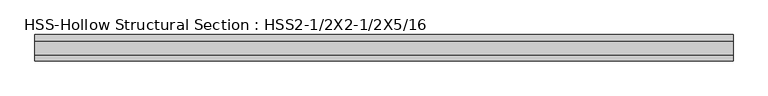
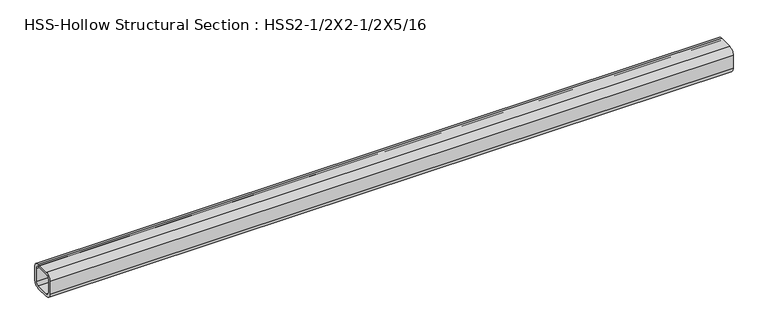
"""IFC4 building model written with IfcOpenShell, lengths in millimetres: beam geometry, HSS-Hollow Structural Section : HSS2-1/2X2-1/2X5/16."""

import ifcopenshell
import ifcopenshell.guid

model = None  # the IFC model being written
_history = None  # IfcOwnerHistory: only IFC2X3 demands one
_inside = {}  # id of a spatial element -> (the spatial element, [elements in it])
_under = {}  # id of a project, library or spatial element -> (it, [spatial elements below it])
_declared = {}  # id of a project -> (the project, [libraries it declares])
_typed = {}  # id of a type object -> (the type object, [elements of that type])
_made_of = {}  # id of a material, layer set ... -> (it, [elements and type objects made of it])


def new_model(schema):
    """Start an empty IFC model of exactly this schema.

    Asked for "IFC4X3", IfcOpenShell would pick the latest addendum, in which some entities
    have other attributes; the version numbers below select the first issue.
    IFC2X3 requires an IfcOwnerHistory on every rooted entity: one is made here for all.
    """
    global model, _history
    if schema == "IFC4X3":
        model = ifcopenshell.file(schema_version=(4, 3, 0, 0))
    else:
        model = ifcopenshell.file(schema=schema)
    _inside.clear()
    _under.clear()
    _declared.clear()
    _typed.clear()
    _made_of.clear()
    _history = None
    if model.schema == "IFC2X3":
        org = make("IfcOrganization", Name="unknown")
        user = make(
            "IfcPersonAndOrganization",
            ThePerson=make("IfcPerson", FamilyName="unknown"),
            TheOrganization=org,
        )
        app = make(
            "IfcApplication",
            ApplicationDeveloper=org,
            Version="unknown",
            ApplicationFullName="unknown",
            ApplicationIdentifier="unknown",
        )
        _history = make(
            "IfcOwnerHistory",
            OwningUser=user,
            OwningApplication=app,
            ChangeAction="ADDED",
            CreationDate=0,
        )
    return model


def make(cls, **values):
    """One entity of the class cls with the attributes given. An attribute that is None is left unset."""
    return model.create_entity(
        cls, **{name: value for name, value in values.items() if value is not None}
    )


def rooted(cls, **values):
    """An entity with a GlobalId (a new one), such as an element, a storey or a relation."""
    return make(cls, GlobalId=ifcopenshell.guid.new(), OwnerHistory=_history, **values)


def si_unit(unit_type, name, prefix=None):
    """IfcSIUnit, for example si_unit("LENGTHUNIT", "METRE", prefix="MILLI")."""
    return make("IfcSIUnit", UnitType=unit_type, Prefix=prefix, Name=name)


def assignment(units):
    """IfcUnitAssignment: the units of a project."""
    return None if units is None else make("IfcUnitAssignment", Units=units)


def point(xyz):
    """IfcCartesianPoint."""
    return None if xyz is None else make("IfcCartesianPoint", Coordinates=xyz)


def direction(xyz):
    """IfcDirection."""
    return None if xyz is None else make("IfcDirection", DirectionRatios=xyz)


def frame(location, z_axis=None, x_axis=None):
    """IfcAxis2Placement3D, a coordinate frame: its origin and axes. An axis left out is left unset."""
    return make(
        "IfcAxis2Placement3D",
        Location=point(location),
        Axis=direction(z_axis),
        RefDirection=direction(x_axis),
    )


def frame_2d(location, x_axis=None):
    """IfcAxis2Placement2D, a coordinate frame in the plane: its origin and x axis."""
    return make(
        "IfcAxis2Placement2D", Location=point(location), RefDirection=direction(x_axis)
    )


def origin():
    """The frame at (0, 0, 0) with its axes left unset."""
    return frame((0.0, 0.0, 0.0))


def place(relative_to, where):
    """IfcLocalPlacement: puts the frame where relative to a parent placement (None: the world)."""
    return make(
        "IfcLocalPlacement", PlacementRelTo=relative_to, RelativePlacement=where
    )


def context(
    kind, dimensions, precision=None, world=None, true_north=None, identifier=None
):
    """IfcGeometricRepresentationContext, for example the 3D "Model" context."""
    return make(
        "IfcGeometricRepresentationContext",
        ContextIdentifier=identifier,
        ContextType=kind,
        CoordinateSpaceDimension=dimensions,
        Precision=precision,
        WorldCoordinateSystem=world,
        TrueNorth=true_north,
    )


def project(units=None, contexts=None):
    """IfcProject with its units and contexts."""
    return rooted(
        "IfcProject",
        Name="project",
        RepresentationContexts=contexts,
        UnitsInContext=assignment(units),
    )


def spatial(cls, under=None, at=None, **own):
    """A site, building, storey or space (cls), placed at a placement, below another one or the project."""
    s = rooted(cls, ObjectPlacement=at, **own)
    if under is not None:
        _under.setdefault(under.id(), (under, []))[1].append(s)
    return s


def polyline(points):
    """IfcPolyline through the points."""
    return make("IfcPolyline", Points=[point(p) for p in points])


def circle_curve(where, radius):
    """IfcCircle in the frame where."""
    return make("IfcCircle", Position=where, Radius=radius)


def trimmed(basis, trim1, trim2, sense, master):
    """IfcTrimmedCurve: the piece of a basis curve between two trims."""
    return make(
        "IfcTrimmedCurve",
        BasisCurve=basis,
        Trim1=trim1,
        Trim2=trim2,
        SenseAgreement=sense,
        MasterRepresentation=master,
    )


def segment(curve, same_sense, transition):
    """IfcCompositeCurveSegment."""
    return make(
        "IfcCompositeCurveSegment",
        Transition=transition,
        SameSense=same_sense,
        ParentCurve=curve,
    )


def composite_curve(segments, self_intersect=None):
    """IfcCompositeCurve: segments joined end to end."""
    return make("IfcCompositeCurve", Segments=segments, SelfIntersect=self_intersect)


def outline(outer, holes=None, kind="AREA"):
    """IfcArbitraryClosedProfileDef: a profile drawn as a closed curve; with holes, ...WithVoids."""
    if holes is None:
        return make("IfcArbitraryClosedProfileDef", ProfileType=kind, OuterCurve=outer)
    return make(
        "IfcArbitraryProfileDefWithVoids",
        ProfileType=kind,
        OuterCurve=outer,
        InnerCurves=holes,
    )


def extrude(swept, where, along, depth):
    """IfcExtrudedAreaSolid: the profile swept, set in the frame where, extruded along a direction by depth."""
    return make(
        "IfcExtrudedAreaSolid",
        SweptArea=swept,
        Position=where,
        ExtrudedDirection=direction(along),
        Depth=depth,
    )


def shape(context_of_items, identifier, shape_type, items):
    """IfcShapeRepresentation: the items that make up one representation, for example the "Body"."""
    return make(
        "IfcShapeRepresentation",
        ContextOfItems=context_of_items,
        RepresentationIdentifier=identifier,
        RepresentationType=shape_type,
        Items=items,
    )


def source(mapping_origin, context_of_items, identifier, shape_type, items):
    """IfcRepresentationMap: a shape defined once, which mapped items show again and again."""
    return make(
        "IfcRepresentationMap",
        MappingOrigin=mapping_origin,
        MappedRepresentation=shape(context_of_items, identifier, shape_type, items),
    )


def transform(
    local_origin,
    x_axis=None,
    y_axis=None,
    z_axis=None,
    scale=None,
    scale2=None,
    scale3=None,
    uniform=True,
):
    """IfcCartesianTransformationOperator3D, or its non-uniform kind. x_axis, y_axis, z_axis: its Axis1, 2, 3."""
    if uniform:
        return make(
            "IfcCartesianTransformationOperator3D",
            Axis1=direction(x_axis),
            Axis2=direction(y_axis),
            LocalOrigin=point(local_origin),
            Scale=scale,
            Axis3=direction(z_axis),
        )
    return make(
        "IfcCartesianTransformationOperator3DnonUniform",
        Axis1=direction(x_axis),
        Axis2=direction(y_axis),
        LocalOrigin=point(local_origin),
        Scale=scale,
        Axis3=direction(z_axis),
        Scale2=scale2,
        Scale3=scale3,
    )


def mapped(mapping_source, mapping_target):
    """IfcMappedItem: shows the shape of a source again, moved by a transform."""
    return make(
        "IfcMappedItem", MappingSource=mapping_source, MappingTarget=mapping_target
    )


def made_of(thing, what):
    """Note that an element or type object is made of a material, layer set ...; save() writes the relation."""
    if what is not None:
        _made_of.setdefault(what.id(), (what, []))[1].append(thing)
    return thing


def element(
    cls,
    number,
    at=None,
    inside=None,
    cuts=None,
    type_object=None,
    material=None,
    context=None,
    identifier="Body",
    shape_type=None,
    held_by="IfcProductDefinitionShape",
    body=None,
    shapes=None,
    **own,
):
    """One element of the class cls, such as IfcWall. Its Tag is "e" and its number.

    at: its placement. inside: the storey or other place that contains it. cuts: it is an
    opening in that element (IfcRelVoidsElement). A single representation is given by context,
    identifier, shape_type and body (its items); several are given by shapes. held_by: the class
    of the entity that holds the representations. save() writes the other relations.
    """
    e = rooted(cls, Tag="e%d" % number, ObjectPlacement=at, **own)
    if body is not None:
        shapes = [shape(context, identifier, shape_type, body)]
    if shapes is not None:
        e.Representation = make(held_by, Representations=shapes)
    if inside is not None:
        _inside.setdefault(inside.id(), (inside, []))[1].append(e)
    if cuts is not None:
        rooted(
            "IfcRelVoidsElement", RelatingBuildingElement=cuts, RelatedOpeningElement=e
        )
    if type_object is not None:
        _typed.setdefault(type_object.id(), (type_object, []))[1].append(e)
    return made_of(e, material)


def aggregate(whole, parts):
    """IfcRelAggregates: a whole, such as a stair, and the parts it consists of."""
    return rooted("IfcRelAggregates", RelatingObject=whole, RelatedObjects=parts)


def save(model, path):
    """Write the relations noted so far, then the file.

    IfcRelAggregates (storeys below a building ...), IfcRelContainedInSpatialStructure (elements
    in a storey), IfcRelDefinesByType, IfcRelAssociatesMaterial and IfcRelDeclares: one each for
    every whole, place, type object, material and project.
    """
    for whole, parts in _under.values():
        aggregate(whole, parts)
    for where, things in _inside.values():
        rooted(
            "IfcRelContainedInSpatialStructure",
            RelatedElements=things,
            RelatingStructure=where,
        )
    for kind, things in _typed.values():
        rooted("IfcRelDefinesByType", RelatedObjects=things, RelatingType=kind)
    for what, things in _made_of.values():
        rooted("IfcRelAssociatesMaterial", RelatedObjects=things, RelatingMaterial=what)
    for by, libraries in _declared.values():
        rooted("IfcRelDeclares", RelatingContext=by, RelatedDefinitions=libraries)
    model.write(path)


def hss_hollow_structural_section_hss2_1_2x2_1_2x5_16_ba63e807(model_context):
    return source(origin(), model_context, "Body", "SweptSolid", [
        extrude(outline(composite_curve([segment(polyline([(31.75, 16.9672), (31.75, -16.9672)]), True, "CONTINUOUS"), segment(trimmed(circle_curve(frame_2d((16.9672, -16.9672)), 14.7828), [point((31.75, -16.9672))], [point((16.9672, -31.75))], False, "CARTESIAN"), True, "CONTINUOUS"), segment(polyline([(16.9672, -31.75), (-16.9672, -31.75)]), True, "CONTINUOUS"), segment(trimmed(circle_curve(frame_2d((-16.9672, -16.9672)), 14.7828), [point((-16.9672, -31.75))], [point((-31.75, -16.9672))], False, "CARTESIAN"), True, "CONTINUOUS"), segment(polyline([(-31.75, -16.9672), (-31.75, 16.9672)]), True, "CONTINUOUS"), segment(trimmed(circle_curve(frame_2d((-16.9672, 16.9672)), 14.7828), [point((-31.75, 16.9672))], [point((-16.9672, 31.75))], False, "CARTESIAN"), True, "CONTINUOUS"), segment(polyline([(-16.9672, 31.75), (16.9672, 31.75)]), True, "CONTINUOUS"), segment(trimmed(circle_curve(frame_2d((16.9672, 16.9672)), 14.7828), [point((16.9672, 31.75))], [point((31.75, 16.9672))], False, "CARTESIAN"), True, "CONTINUOUS")], self_intersect=False), holes=[composite_curve([segment(trimmed(circle_curve(frame_2d((-16.9672, 16.9672)), 7.3914), [point((-16.9672, 24.3586))], [point((-24.3586, 16.9672))], True, "CARTESIAN"), True, "CONTINUOUS"), segment(polyline([(-24.3586, 16.9672), (-24.3586, -16.9672)]), True, "CONTINUOUS"), segment(trimmed(circle_curve(frame_2d((-16.9672, -16.9672)), 7.3914), [point((-24.3586, -16.9672))], [point((-16.9672, -24.3586))], True, "CARTESIAN"), True, "CONTINUOUS"), segment(polyline([(-16.9672, -24.3586), (16.9672, -24.3586)]), True, "CONTINUOUS"), segment(trimmed(circle_curve(frame_2d((16.9672, -16.9672)), 7.3914), [point((16.9672, -24.3586))], [point((24.3586, -16.9672))], True, "CARTESIAN"), True, "CONTINUOUS"), segment(polyline([(24.3586, -16.9672), (24.3586, 16.9672)]), True, "CONTINUOUS"), segment(trimmed(circle_curve(frame_2d((16.9672, 16.9672)), 7.3914), [point((24.3586, 16.9672))], [point((16.9672, 24.3586))], True, "CARTESIAN"), True, "CONTINUOUS"), segment(polyline([(16.9672, 24.3586), (-16.9672, 24.3586)]), True, "CONTINUOUS")], self_intersect=False)]), frame((-831.85, 0.0, 0.0), z_axis=(1.0, 0.0, 0.0), x_axis=(0.0, 1.0, 0.0)), (0.0, 0.0, 1.0), 1682.877),
    ])


if __name__ == "__main__":
    model = new_model("IFC4")
    model_context = context("Model", 3, world=origin())
    ifc_project = project(units=[si_unit("LENGTHUNIT", "METRE", prefix="MILLI")], contexts=[model_context])
    site = spatial("IfcSite", under=ifc_project)
    building = spatial("IfcBuilding", under=site)
    placement = place(None, origin())
    hss_hollow_structural_section_hss2_1_2x2_1_2x5_16_shape = hss_hollow_structural_section_hss2_1_2x2_1_2x5_16_ba63e807(model_context)
    element("IfcBeam", 1, ObjectType="HSS-Hollow Structural Section : HSS2-1/2X2-1/2X5/16", at=placement, inside=building, context=model_context, shape_type="MappedRepresentation", body=[
        mapped(hss_hollow_structural_section_hss2_1_2x2_1_2x5_16_shape, transform((0.0, 0.0, 0.0), x_axis=(1.0, 0.0, 0.0), y_axis=(0.0, 1.0, 0.0), z_axis=(0.0, 0.0, 1.0))),
    ])
    save(model, "model.ifc")

# Revit data of these elements
# Type "HSS-Hollow Structural Section : HSS2-1/2X2-1/2X5/16"
#   Assembly Code = "B10"
#   Shape = "Square"
#   W = 8.4
#   Ht = 0' - 2 1/2"
#   Length [instance default] = 5' - 0"
#   b = 0' - 2 1/2"
#   kr = 0' - 0.582"
#   t = 0' - 0.291"
#   A = 0.0163194 SF
#   Structural Material [instance default] = Steel ASTM A500, Grade B, Rectangular and Square
# Element 1 (IfcBeam, "HSS-Hollow Structural Section : HSS2-1/2X2-1/2X5/16")
#   Materials on its faces: "Steel ASTM A500, Grade B, Rectangular and Square"
# Materials
#   "Steel ASTM A500, Grade B, Rectangular and Square": class "Metal", colour RGB 199 199 199, transparency 0, Description = "Carbon steel", Cost = 0
